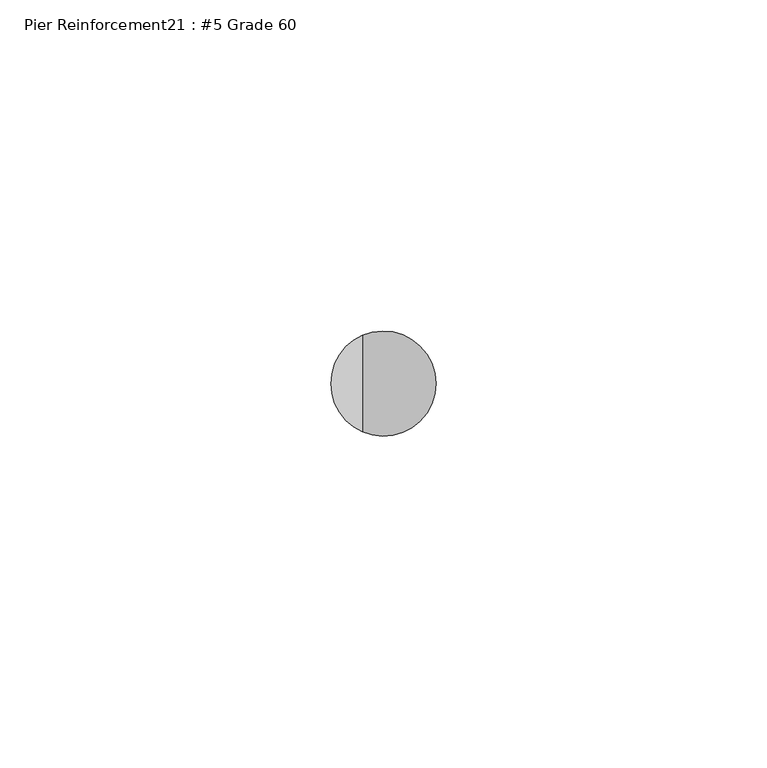
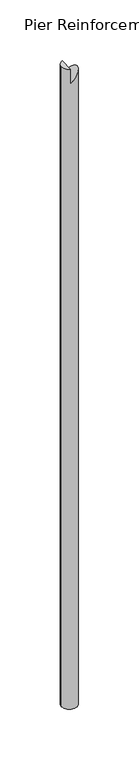
"""IFC4 building model written with IfcOpenShell, lengths in millimetres: proxy geometry, Pier Reinforcement21 : #5 Grade 60."""

from ifc_helpers import new_model, si_unit, frame, origin, place, context, project, spatial, circle_curve, ellipse_curve, source, transform, mapped, element, save
from ifc_brep_helpers import plane_surface, cylinder_surface, advanced_brep


def pier_reinforcement21_5_grade_60_f625620a(model_context):
    return source(origin(), model_context, "Body", "AdvancedBrep", [
        advanced_brep(
        [(590218.1172365, -534096.6663841, -47.625), (590222.8797365, -534103.941223, -47.625), (590222.8797365, -534089.3915452, -47.625), (590218.1172365, -534096.6663841, -733.425), (590233.9922365, -534096.6663841, -733.425), (590233.9922365, -534096.6663841, -52.3875), (590222.8797365, -534103.941223, -63.5), (590222.8797365, -534089.3915452, -63.5)],
        [
            (0, 1, circle_curve(frame((590226.0547365, -534096.6663841, -47.625), z_axis=(0.0, 0.0, 1.0), x_axis=(1.0, 0.0, 0.0)), 7.9375)),
            (1, 2),
            (2, 0, circle_curve(frame((590226.0547365, -534096.6663841, -47.625), z_axis=(0.0, 0.0, 1.0), x_axis=(1.0, 0.0, 0.0)), 7.9375)),
            (3, 4, circle_curve(frame((590226.0547365, -534096.6663841, -733.425), z_axis=(0.0, 0.0, -1.0), x_axis=(1.0, 0.0, 0.0)), 7.9375)),
            (4, 3, circle_curve(frame((590226.0547365, -534096.6663841, -733.425), z_axis=(0.0, 0.0, -1.0), x_axis=(1.0, 0.0, 0.0)), 7.9375)),
            (4, 5),
            (5, 6, ellipse_curve(frame((590226.0547365, -534096.6663841, -60.325), z_axis=(0.707106781186547, 0.0, -0.7071067811865481), x_axis=(0.7071067811865481, 0.0, 0.7071067811865468)), 11.2253202, 7.9375)),
            (6, 1),
            (0, 3),
            (2, 7),
            (7, 5, ellipse_curve(frame((590226.0547365, -534096.6663841, -60.325), z_axis=(0.707106781186547, 0.0, -0.7071067811865481), x_axis=(0.7071067811865481, 0.0, 0.7071067811865468)), 11.2253202, 7.9375)),
            (6, 7),
        ],
        [
            plane_surface(frame((590233.9922365, -534096.6663841, -47.625), z_axis=(0.0, 0.0, 1.0), x_axis=(0.0, 1.0, 0.0))),
            plane_surface(frame((590233.9922365, -534096.6663841, -733.425), z_axis=(0.0, 0.0, -1.0), x_axis=(0.0, -1.0, 0.0))),
            cylinder_surface(frame((590226.0547365, -534096.6663841, -733.425), z_axis=(0.0, 0.0, 1.0), x_axis=(1.0, 0.0, 0.0)), 7.9375),
            plane_surface(frame((590222.8797365, -534128.4163841, -47.625), z_axis=(1.0, 0.0, 0.0), x_axis=(0.0, 1.0, 0.0))),
            plane_surface(frame((590222.8797365, -534128.4163841, -63.5), z_axis=(-0.707106781186547, 0.0, 0.7071067811865481), x_axis=(0.0, 1.0, 0.0))),
        ],
        [
            (0, [[1, 2, 3]]),
            (1, [[4, 5]]),
            (2, [[-5, 6, 7, 8, -1, 9]]),
            (2, [[-4, -9, -3, 10, 11, -6]]),
            (3, [[12, -10, -2, -8]]),
            (4, [[-12, -7, -11]]),
        ],
    ),
    ])


if __name__ == "__main__":
    model = new_model("IFC4")
    model_context = context("Model", 3, world=origin())
    ifc_project = project(units=[si_unit("LENGTHUNIT", "METRE", prefix="MILLI")], contexts=[model_context])
    site = spatial("IfcSite", under=ifc_project)
    building = spatial("IfcBuilding", under=site)
    placement = place(None, origin())
    pier_reinforcement21_5_grade_60_shape = pier_reinforcement21_5_grade_60_f625620a(model_context)
    element("IfcBuildingElementProxy", 1, Name="Pier Reinforcement21 : #5 Grade 60", ObjectType="Pier Reinforcement21 : #5 Grade 60", at=placement, inside=building, context=model_context, shape_type="MappedRepresentation", body=[
        mapped(pier_reinforcement21_5_grade_60_shape, transform((0.0, 0.0, 0.0), x_axis=(1.0, 0.0, 0.0), y_axis=(0.0, 1.0, 0.0), z_axis=(0.0, 0.0, 1.0))),
    ])
    save(model, "model.ifc")

# Revit data of these elements
# Element 1 (IfcBuildingElementProxy, "Pier Reinforcement21 : #5 Grade 60")
#   Materials on its faces: "#4 GR. 60 REINF. @ 16\" O.C. EW."
# Materials
#   "#4 GR. 60 REINF. @ 16\" O.C. EW.": class "Generic", colour RGB 84 83 81, transparency 0, Cost = 0
